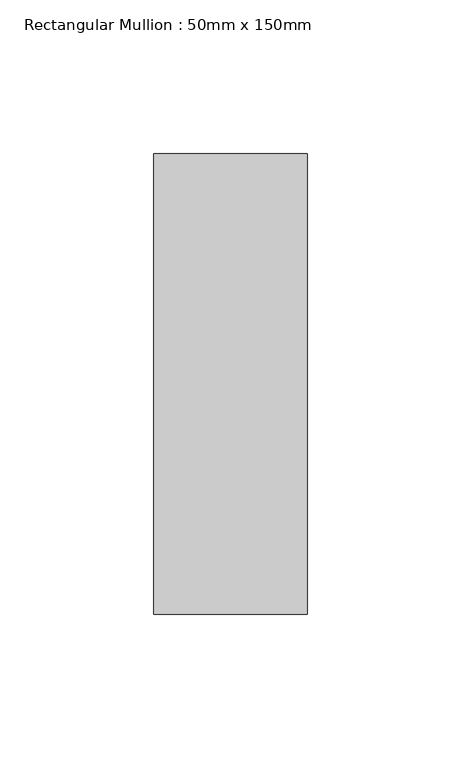
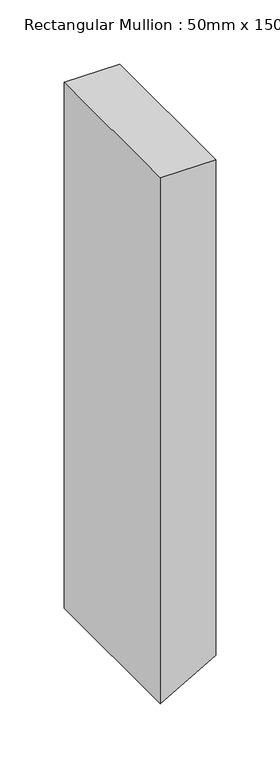
"""IFC4 building model written with IfcOpenShell, lengths in millimetres: member geometry, Rectangular Mullion : 50mm x 150mm."""

import ifcopenshell
import ifcopenshell.guid

model = None  # the IFC model being written
_history = None  # IfcOwnerHistory: only IFC2X3 demands one
_inside = {}  # id of a spatial element -> (the spatial element, [elements in it])
_under = {}  # id of a project, library or spatial element -> (it, [spatial elements below it])
_declared = {}  # id of a project -> (the project, [libraries it declares])
_typed = {}  # id of a type object -> (the type object, [elements of that type])
_made_of = {}  # id of a material, layer set ... -> (it, [elements and type objects made of it])


def new_model(schema):
    """Start an empty IFC model of exactly this schema.

    Asked for "IFC4X3", IfcOpenShell would pick the latest addendum, in which some entities
    have other attributes; the version numbers below select the first issue.
    IFC2X3 requires an IfcOwnerHistory on every rooted entity: one is made here for all.
    """
    global model, _history
    if schema == "IFC4X3":
        model = ifcopenshell.file(schema_version=(4, 3, 0, 0))
    else:
        model = ifcopenshell.file(schema=schema)
    _inside.clear()
    _under.clear()
    _declared.clear()
    _typed.clear()
    _made_of.clear()
    _history = None
    if model.schema == "IFC2X3":
        org = make("IfcOrganization", Name="unknown")
        user = make(
            "IfcPersonAndOrganization",
            ThePerson=make("IfcPerson", FamilyName="unknown"),
            TheOrganization=org,
        )
        app = make(
            "IfcApplication",
            ApplicationDeveloper=org,
            Version="unknown",
            ApplicationFullName="unknown",
            ApplicationIdentifier="unknown",
        )
        _history = make(
            "IfcOwnerHistory",
            OwningUser=user,
            OwningApplication=app,
            ChangeAction="ADDED",
            CreationDate=0,
        )
    return model


def make(cls, **values):
    """One entity of the class cls with the attributes given. An attribute that is None is left unset."""
    return model.create_entity(
        cls, **{name: value for name, value in values.items() if value is not None}
    )


def rooted(cls, **values):
    """An entity with a GlobalId (a new one), such as an element, a storey or a relation."""
    return make(cls, GlobalId=ifcopenshell.guid.new(), OwnerHistory=_history, **values)


def si_unit(unit_type, name, prefix=None):
    """IfcSIUnit, for example si_unit("LENGTHUNIT", "METRE", prefix="MILLI")."""
    return make("IfcSIUnit", UnitType=unit_type, Prefix=prefix, Name=name)


def assignment(units):
    """IfcUnitAssignment: the units of a project."""
    return None if units is None else make("IfcUnitAssignment", Units=units)


def point(xyz):
    """IfcCartesianPoint."""
    return None if xyz is None else make("IfcCartesianPoint", Coordinates=xyz)


def direction(xyz):
    """IfcDirection."""
    return None if xyz is None else make("IfcDirection", DirectionRatios=xyz)


def frame(location, z_axis=None, x_axis=None):
    """IfcAxis2Placement3D, a coordinate frame: its origin and axes. An axis left out is left unset."""
    return make(
        "IfcAxis2Placement3D",
        Location=point(location),
        Axis=direction(z_axis),
        RefDirection=direction(x_axis),
    )


def origin():
    """The frame at (0, 0, 0) with its axes left unset."""
    return frame((0.0, 0.0, 0.0))


def place(relative_to, where):
    """IfcLocalPlacement: puts the frame where relative to a parent placement (None: the world)."""
    return make(
        "IfcLocalPlacement", PlacementRelTo=relative_to, RelativePlacement=where
    )


def context(
    kind, dimensions, precision=None, world=None, true_north=None, identifier=None
):
    """IfcGeometricRepresentationContext, for example the 3D "Model" context."""
    return make(
        "IfcGeometricRepresentationContext",
        ContextIdentifier=identifier,
        ContextType=kind,
        CoordinateSpaceDimension=dimensions,
        Precision=precision,
        WorldCoordinateSystem=world,
        TrueNorth=true_north,
    )


def project(units=None, contexts=None):
    """IfcProject with its units and contexts."""
    return rooted(
        "IfcProject",
        Name="project",
        RepresentationContexts=contexts,
        UnitsInContext=assignment(units),
    )


def spatial(cls, under=None, at=None, **own):
    """A site, building, storey or space (cls), placed at a placement, below another one or the project."""
    s = rooted(cls, ObjectPlacement=at, **own)
    if under is not None:
        _under.setdefault(under.id(), (under, []))[1].append(s)
    return s


def polyline(points):
    """IfcPolyline through the points."""
    return make("IfcPolyline", Points=[point(p) for p in points])


def outline(outer, holes=None, kind="AREA"):
    """IfcArbitraryClosedProfileDef: a profile drawn as a closed curve; with holes, ...WithVoids."""
    if holes is None:
        return make("IfcArbitraryClosedProfileDef", ProfileType=kind, OuterCurve=outer)
    return make(
        "IfcArbitraryProfileDefWithVoids",
        ProfileType=kind,
        OuterCurve=outer,
        InnerCurves=holes,
    )


def extrude(swept, where, along, depth):
    """IfcExtrudedAreaSolid: the profile swept, set in the frame where, extruded along a direction by depth."""
    return make(
        "IfcExtrudedAreaSolid",
        SweptArea=swept,
        Position=where,
        ExtrudedDirection=direction(along),
        Depth=depth,
    )


def shape(context_of_items, identifier, shape_type, items):
    """IfcShapeRepresentation: the items that make up one representation, for example the "Body"."""
    return make(
        "IfcShapeRepresentation",
        ContextOfItems=context_of_items,
        RepresentationIdentifier=identifier,
        RepresentationType=shape_type,
        Items=items,
    )


def source(mapping_origin, context_of_items, identifier, shape_type, items):
    """IfcRepresentationMap: a shape defined once, which mapped items show again and again."""
    return make(
        "IfcRepresentationMap",
        MappingOrigin=mapping_origin,
        MappedRepresentation=shape(context_of_items, identifier, shape_type, items),
    )


def transform(
    local_origin,
    x_axis=None,
    y_axis=None,
    z_axis=None,
    scale=None,
    scale2=None,
    scale3=None,
    uniform=True,
):
    """IfcCartesianTransformationOperator3D, or its non-uniform kind. x_axis, y_axis, z_axis: its Axis1, 2, 3."""
    if uniform:
        return make(
            "IfcCartesianTransformationOperator3D",
            Axis1=direction(x_axis),
            Axis2=direction(y_axis),
            LocalOrigin=point(local_origin),
            Scale=scale,
            Axis3=direction(z_axis),
        )
    return make(
        "IfcCartesianTransformationOperator3DnonUniform",
        Axis1=direction(x_axis),
        Axis2=direction(y_axis),
        LocalOrigin=point(local_origin),
        Scale=scale,
        Axis3=direction(z_axis),
        Scale2=scale2,
        Scale3=scale3,
    )


def mapped(mapping_source, mapping_target):
    """IfcMappedItem: shows the shape of a source again, moved by a transform."""
    return make(
        "IfcMappedItem", MappingSource=mapping_source, MappingTarget=mapping_target
    )


def made_of(thing, what):
    """Note that an element or type object is made of a material, layer set ...; save() writes the relation."""
    if what is not None:
        _made_of.setdefault(what.id(), (what, []))[1].append(thing)
    return thing


def element(
    cls,
    number,
    at=None,
    inside=None,
    cuts=None,
    type_object=None,
    material=None,
    context=None,
    identifier="Body",
    shape_type=None,
    held_by="IfcProductDefinitionShape",
    body=None,
    shapes=None,
    **own,
):
    """One element of the class cls, such as IfcWall. Its Tag is "e" and its number.

    at: its placement. inside: the storey or other place that contains it. cuts: it is an
    opening in that element (IfcRelVoidsElement). A single representation is given by context,
    identifier, shape_type and body (its items); several are given by shapes. held_by: the class
    of the entity that holds the representations. save() writes the other relations.
    """
    e = rooted(cls, Tag="e%d" % number, ObjectPlacement=at, **own)
    if body is not None:
        shapes = [shape(context, identifier, shape_type, body)]
    if shapes is not None:
        e.Representation = make(held_by, Representations=shapes)
    if inside is not None:
        _inside.setdefault(inside.id(), (inside, []))[1].append(e)
    if cuts is not None:
        rooted(
            "IfcRelVoidsElement", RelatingBuildingElement=cuts, RelatedOpeningElement=e
        )
    if type_object is not None:
        _typed.setdefault(type_object.id(), (type_object, []))[1].append(e)
    return made_of(e, material)


def aggregate(whole, parts):
    """IfcRelAggregates: a whole, such as a stair, and the parts it consists of."""
    return rooted("IfcRelAggregates", RelatingObject=whole, RelatedObjects=parts)


def save(model, path):
    """Write the relations noted so far, then the file.

    IfcRelAggregates (storeys below a building ...), IfcRelContainedInSpatialStructure (elements
    in a storey), IfcRelDefinesByType, IfcRelAssociatesMaterial and IfcRelDeclares: one each for
    every whole, place, type object, material and project.
    """
    for whole, parts in _under.values():
        aggregate(whole, parts)
    for where, things in _inside.values():
        rooted(
            "IfcRelContainedInSpatialStructure",
            RelatedElements=things,
            RelatingStructure=where,
        )
    for kind, things in _typed.values():
        rooted("IfcRelDefinesByType", RelatedObjects=things, RelatingType=kind)
    for what, things in _made_of.values():
        rooted("IfcRelAssociatesMaterial", RelatedObjects=things, RelatingMaterial=what)
    for by, libraries in _declared.values():
        rooted("IfcRelDeclares", RelatingContext=by, RelatedDefinitions=libraries)
    model.write(path)


def rectangular_mullion_50mm_x_150mm_d4c3fc6e(model_context):
    return source(origin(), model_context, "Body", "SweptSolid", [
        extrude(outline(polyline([(0.0, 25.0), (0.0, -25.0), (-501.2276186, -25.0), (-472.3601051, 25.0), (0.0, 25.0)])), frame((0.0, -75.0, 0.0), z_axis=(0.0, 1.0, 0.0), x_axis=(0.0, 0.0, 1.0)), (0.0, 0.0, 1.0), 150.0),
    ])


if __name__ == "__main__":
    model = new_model("IFC4")
    model_context = context("Model", 3, world=origin())
    ifc_project = project(units=[si_unit("LENGTHUNIT", "METRE", prefix="MILLI")], contexts=[model_context])
    site = spatial("IfcSite", under=ifc_project)
    building = spatial("IfcBuilding", under=site)
    placement = place(None, origin())
    rectangular_mullion_50mm_x_150mm_shape = rectangular_mullion_50mm_x_150mm_d4c3fc6e(model_context)
    element("IfcMember", 1, ObjectType="Rectangular Mullion : 50mm x 150mm", at=placement, inside=building, context=model_context, shape_type="MappedRepresentation", body=[
        mapped(rectangular_mullion_50mm_x_150mm_shape, transform((0.0, 0.0, 0.0), x_axis=(1.0, 0.0, 0.0), y_axis=(0.0, 1.0, 0.0), z_axis=(0.0, 0.0, 1.0))),
    ])
    save(model, "model.ifc")

# Revit data of these elements
# Type "Rectangular Mullion : 50mm x 150mm"
#   built-in parameter 1007304 = 0.492126 (stored number, unit not read)
#   built-in parameter 1007301 = 0.082021 (stored number, unit not read)
#   built-in parameter 1007300 = 0.082021 (stored number, unit not read)
# Element 1 (IfcMember, "Rectangular Mullion : 50mm x 150mm")
#   Materials on its faces: "Aluminum"
# Materials
#   "Aluminum": class "Metal", colour RGB 247 247 247, transparency 0, Description = "Aluminum 6061", Cost = 0
